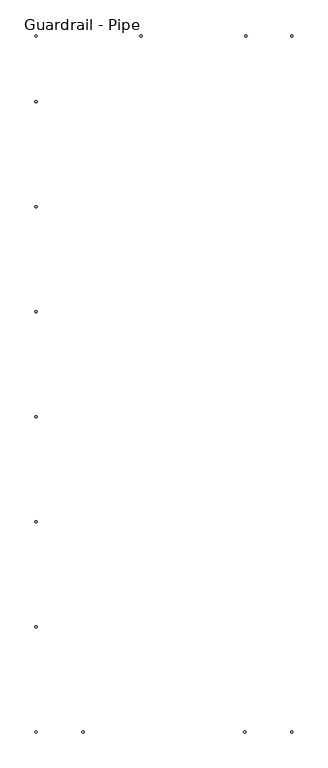
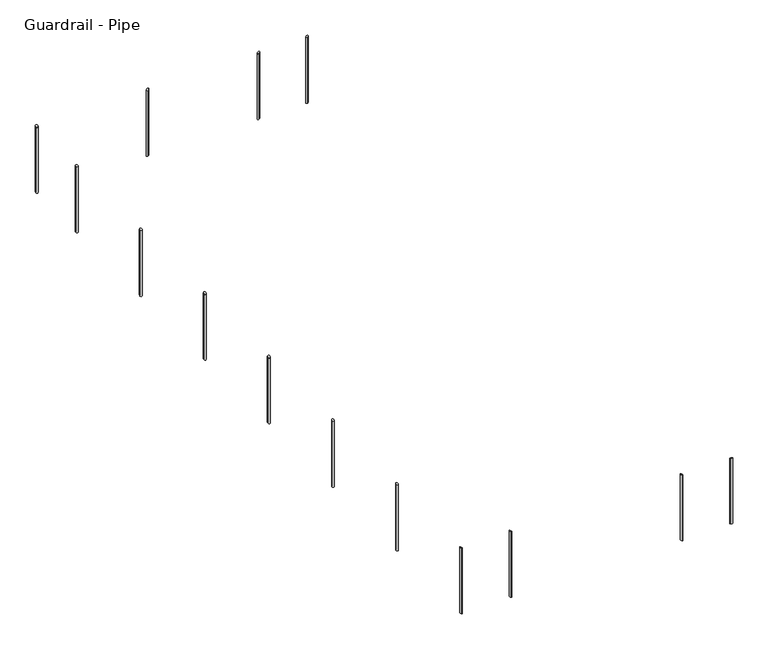
"""IFC4 building model written with IfcOpenShell, lengths in millimetres: railing geometry, Guardrail - Pipe."""

from ifc_helpers import new_model, si_unit, frame, origin, place, context, project, spatial, ellipse_curve, source, transform, mapped, element, save
from ifc_brep_helpers import plane_surface, cylinder_surface, advanced_brep


def guardrail_pipe_e2f870d2(model_context):
    return source(origin(), model_context, "Body", "AdvancedBrep", [
        advanced_brep(
        [(13413.9313551, 29924.3, 8077.2), (13413.9313551, 29924.3, 7315.2), (13413.9313551, 29949.7, 7315.2), (13413.9313551, 29949.7, 8077.2)],
        [
            (0, 1),
            (1, 2, ellipse_curve(frame((13413.9313551, 29937.0, 7315.2), z_axis=(-0.536857935986758, 0.0, 0.8436726596068158), x_axis=(0.8436726596068159, 0.0, 0.536857935986758)), 15.0532317, 12.7)),
            (2, 3),
            (3, 0, ellipse_curve(frame((13413.9313551, 29937.0, 8077.2), z_axis=(0.5368579359867546, 0.0, -0.8436726596068179), x_axis=(0.843672659606818, 0.0, 0.5368579359867547)), 15.0532317, 12.7)),
            (0, 3, ellipse_curve(frame((13413.9313551, 29937.0, 8077.2), z_axis=(0.5368579359867546, 0.0, -0.8436726596068179), x_axis=(0.843672659606818, 0.0, 0.5368579359867547)), 15.0532317, 12.7)),
            (2, 1, ellipse_curve(frame((13413.9313551, 29937.0, 7315.2), z_axis=(-0.536857935986758, 0.0, 0.8436726596068158), x_axis=(0.8436726596068159, 0.0, 0.536857935986758)), 15.0532317, 12.7)),
        ],
        [
            cylinder_surface(frame((13413.9313551, 29937.0, 7086.6), z_axis=(0.0, 0.0, 1.0), x_axis=(0.0, 1.0, 0.0)), 12.7),
            plane_surface(frame((13439.3313551, 29962.4, 8093.3628938), z_axis=(-0.5368579359867546, 0.0, 0.8436726596068179), x_axis=(0.0, -1.0, 0.0))),
            plane_surface(frame((13388.5313551, 29962.4, 7299.0371062), z_axis=(0.536857935986758, 0.0, -0.8436726596068158), x_axis=(0.0, -1.0, 0.0))),
        ],
        [
            (0, [[1, 2, 3, 4]]),
            (0, [[-1, 5, -3, 6]]),
            (1, [[-4, -5]]),
            (2, [[-2, -6]]),
        ],
    ),
        advanced_brep(
        [(12194.7313551, 29924.3, 8077.2), (12194.7313551, 29924.3, 7315.2), (12194.7313551, 29949.7, 7315.2), (12194.7313551, 29949.7, 8077.2)],
        [
            (0, 1),
            (1, 2, ellipse_curve(frame((12194.7313551, 29937.0, 7315.2), z_axis=(-0.536857935986758, 0.0, 0.8436726596068158), x_axis=(0.8436726596068159, 0.0, 0.536857935986758)), 15.0532317, 12.7)),
            (2, 3),
            (3, 0, ellipse_curve(frame((12194.7313551, 29937.0, 8077.2), z_axis=(0.5368579359867546, 0.0, -0.8436726596068179), x_axis=(0.843672659606818, 0.0, 0.5368579359867547)), 15.0532317, 12.7)),
            (0, 3, ellipse_curve(frame((12194.7313551, 29937.0, 8077.2), z_axis=(0.5368579359867546, 0.0, -0.8436726596068179), x_axis=(0.843672659606818, 0.0, 0.5368579359867547)), 15.0532317, 12.7)),
            (2, 1, ellipse_curve(frame((12194.7313551, 29937.0, 7315.2), z_axis=(-0.536857935986758, 0.0, 0.8436726596068158), x_axis=(0.8436726596068159, 0.0, 0.536857935986758)), 15.0532317, 12.7)),
        ],
        [
            cylinder_surface(frame((12194.7313551, 29937.0, 7086.6), z_axis=(0.0, 0.0, 1.0), x_axis=(0.0, 1.0, 0.0)), 12.7),
            plane_surface(frame((12220.1313551, 29962.4, 8093.3628938), z_axis=(-0.5368579359867546, 0.0, 0.8436726596068179), x_axis=(0.0, -1.0, 0.0))),
            plane_surface(frame((12169.3313551, 29962.4, 7299.0371062), z_axis=(0.536857935986758, 0.0, -0.8436726596068158), x_axis=(0.0, -1.0, 0.0))),
        ],
        [
            (0, [[1, 2, 3, 4]]),
            (0, [[-1, 5, -3, 6]]),
            (1, [[-4, -5]]),
            (2, [[-2, -6]]),
        ],
    ),
        advanced_brep(
        [(10988.2313551, 29175.0, 8077.2), (10988.2313551, 29175.0, 7315.2), (10962.8313551, 29175.0, 7315.2), (10962.8313551, 29175.0, 8077.2)],
        [
            (0, 1),
            (1, 2, ellipse_curve(frame((10975.5313551, 29175.0, 7315.2), z_axis=(0.0, -0.536857935986758, 0.8436726596068158), x_axis=(0.0, 0.8436726596068159, 0.536857935986758)), 15.0532317, 12.7)),
            (2, 3),
            (3, 0, ellipse_curve(frame((10975.5313551, 29175.0, 8077.2), z_axis=(0.0, 0.5368579359867546, -0.8436726596068179), x_axis=(0.0, 0.843672659606818, 0.5368579359867547)), 15.0532317, 12.7)),
            (0, 3, ellipse_curve(frame((10975.5313551, 29175.0, 8077.2), z_axis=(0.0, 0.5368579359867546, -0.8436726596068179), x_axis=(0.0, 0.843672659606818, 0.5368579359867547)), 15.0532317, 12.7)),
            (2, 1, ellipse_curve(frame((10975.5313551, 29175.0, 7315.2), z_axis=(0.0, -0.536857935986758, 0.8436726596068158), x_axis=(0.0, 0.8436726596068159, 0.536857935986758)), 15.0532317, 12.7)),
        ],
        [
            cylinder_surface(frame((10975.5313551, 29175.0, 7086.6), z_axis=(0.0, 0.0, 1.0), x_axis=(-1.0, 0.0, 0.0)), 12.7),
            plane_surface(frame((10950.1313551, 29200.4, 8093.3628938), z_axis=(0.0, -0.5368579359867546, 0.8436726596068179), x_axis=(1.0, 0.0, 0.0))),
            plane_surface(frame((10950.1313551, 29149.6, 7299.0371062), z_axis=(0.0, 0.536857935986758, -0.8436726596068158), x_axis=(1.0, 0.0, 0.0))),
        ],
        [
            (0, [[1, 2, 3, 4]]),
            (0, [[-1, 5, -3, 6]]),
            (1, [[-4, -5]]),
            (2, [[-2, -6]]),
        ],
    ),
        advanced_brep(
        [(10988.2313551, 27955.8, 8077.2), (10988.2313551, 27955.8, 7315.2), (10962.8313551, 27955.8, 7315.2), (10962.8313551, 27955.8, 8077.2)],
        [
            (0, 1),
            (1, 2, ellipse_curve(frame((10975.5313551, 27955.8, 7315.2), z_axis=(0.0, -0.536857935986758, 0.8436726596068158), x_axis=(0.0, 0.8436726596068159, 0.536857935986758)), 15.0532317, 12.7)),
            (2, 3),
            (3, 0, ellipse_curve(frame((10975.5313551, 27955.8, 8077.2), z_axis=(0.0, 0.5368579359867546, -0.8436726596068179), x_axis=(0.0, 0.843672659606818, 0.5368579359867547)), 15.0532317, 12.7)),
            (0, 3, ellipse_curve(frame((10975.5313551, 27955.8, 8077.2), z_axis=(0.0, 0.5368579359867546, -0.8436726596068179), x_axis=(0.0, 0.843672659606818, 0.5368579359867547)), 15.0532317, 12.7)),
            (2, 1, ellipse_curve(frame((10975.5313551, 27955.8, 7315.2), z_axis=(0.0, -0.536857935986758, 0.8436726596068158), x_axis=(0.0, 0.8436726596068159, 0.536857935986758)), 15.0532317, 12.7)),
        ],
        [
            cylinder_surface(frame((10975.5313551, 27955.8, 7086.6), z_axis=(0.0, 0.0, 1.0), x_axis=(-1.0, 0.0, 0.0)), 12.7),
            plane_surface(frame((10950.1313551, 27981.2, 8093.3628938), z_axis=(0.0, -0.5368579359867546, 0.8436726596068179), x_axis=(1.0, 0.0, 0.0))),
            plane_surface(frame((10950.1313551, 27930.4, 7299.0371062), z_axis=(0.0, 0.536857935986758, -0.8436726596068158), x_axis=(1.0, 0.0, 0.0))),
        ],
        [
            (0, [[1, 2, 3, 4]]),
            (0, [[-1, 5, -3, 6]]),
            (1, [[-4, -5]]),
            (2, [[-2, -6]]),
        ],
    ),
        advanced_brep(
        [(10988.2313551, 26736.6, 8077.2), (10988.2313551, 26736.6, 7315.2), (10962.8313551, 26736.6, 7315.2), (10962.8313551, 26736.6, 8077.2)],
        [
            (0, 1),
            (1, 2, ellipse_curve(frame((10975.5313551, 26736.6, 7315.2), z_axis=(0.0, -0.536857935986758, 0.8436726596068158), x_axis=(0.0, 0.8436726596068159, 0.536857935986758)), 15.0532317, 12.7)),
            (2, 3),
            (3, 0, ellipse_curve(frame((10975.5313551, 26736.6, 8077.2), z_axis=(0.0, 0.5368579359867546, -0.8436726596068179), x_axis=(0.0, 0.843672659606818, 0.5368579359867547)), 15.0532317, 12.7)),
            (0, 3, ellipse_curve(frame((10975.5313551, 26736.6, 8077.2), z_axis=(0.0, 0.5368579359867546, -0.8436726596068179), x_axis=(0.0, 0.843672659606818, 0.5368579359867547)), 15.0532317, 12.7)),
            (2, 1, ellipse_curve(frame((10975.5313551, 26736.6, 7315.2), z_axis=(0.0, -0.536857935986758, 0.8436726596068158), x_axis=(0.0, 0.8436726596068159, 0.536857935986758)), 15.0532317, 12.7)),
        ],
        [
            cylinder_surface(frame((10975.5313551, 26736.6, 7086.6), z_axis=(0.0, 0.0, 1.0), x_axis=(-1.0, 0.0, 0.0)), 12.7),
            plane_surface(frame((10950.1313551, 26762.0, 8093.3628938), z_axis=(0.0, -0.5368579359867546, 0.8436726596068179), x_axis=(1.0, 0.0, 0.0))),
            plane_surface(frame((10950.1313551, 26711.2, 7299.0371062), z_axis=(0.0, 0.536857935986758, -0.8436726596068158), x_axis=(1.0, 0.0, 0.0))),
        ],
        [
            (0, [[1, 2, 3, 4]]),
            (0, [[-1, 5, -3, 6]]),
            (1, [[-4, -5]]),
            (2, [[-2, -6]]),
        ],
    ),
        advanced_brep(
        [(10988.2313551, 25517.4, 8077.2), (10988.2313551, 25517.4, 7315.2), (10962.8313551, 25517.4, 7315.2), (10962.8313551, 25517.4, 8077.2)],
        [
            (0, 1),
            (1, 2, ellipse_curve(frame((10975.5313551, 25517.4, 7315.2), z_axis=(0.0, -0.536857935986758, 0.8436726596068158), x_axis=(0.0, 0.8436726596068159, 0.536857935986758)), 15.0532317, 12.7)),
            (2, 3),
            (3, 0, ellipse_curve(frame((10975.5313551, 25517.4, 8077.2), z_axis=(0.0, 0.5368579359867546, -0.8436726596068179), x_axis=(0.0, 0.843672659606818, 0.5368579359867547)), 15.0532317, 12.7)),
            (0, 3, ellipse_curve(frame((10975.5313551, 25517.4, 8077.2), z_axis=(0.0, 0.5368579359867546, -0.8436726596068179), x_axis=(0.0, 0.843672659606818, 0.5368579359867547)), 15.0532317, 12.7)),
            (2, 1, ellipse_curve(frame((10975.5313551, 25517.4, 7315.2), z_axis=(0.0, -0.536857935986758, 0.8436726596068158), x_axis=(0.0, 0.8436726596068159, 0.536857935986758)), 15.0532317, 12.7)),
        ],
        [
            cylinder_surface(frame((10975.5313551, 25517.4, 7086.6), z_axis=(0.0, 0.0, 1.0), x_axis=(-1.0, 0.0, 0.0)), 12.7),
            plane_surface(frame((10950.1313551, 25542.8, 8093.3628938), z_axis=(0.0, -0.5368579359867546, 0.8436726596068179), x_axis=(1.0, 0.0, 0.0))),
            plane_surface(frame((10950.1313551, 25492.0, 7299.0371062), z_axis=(0.0, 0.536857935986758, -0.8436726596068158), x_axis=(1.0, 0.0, 0.0))),
        ],
        [
            (0, [[1, 2, 3, 4]]),
            (0, [[-1, 5, -3, 6]]),
            (1, [[-4, -5]]),
            (2, [[-2, -6]]),
        ],
    ),
        advanced_brep(
        [(10988.2313551, 24298.2, 8077.2), (10988.2313551, 24298.2, 7315.2), (10962.8313551, 24298.2, 7315.2), (10962.8313551, 24298.2, 8077.2)],
        [
            (0, 1),
            (1, 2, ellipse_curve(frame((10975.5313551, 24298.2, 7315.2), z_axis=(0.0, -0.536857935986758, 0.8436726596068158), x_axis=(0.0, 0.8436726596068159, 0.536857935986758)), 15.0532317, 12.7)),
            (2, 3),
            (3, 0, ellipse_curve(frame((10975.5313551, 24298.2, 8077.2), z_axis=(0.0, 0.5368579359867546, -0.8436726596068179), x_axis=(0.0, 0.843672659606818, 0.5368579359867547)), 15.0532317, 12.7)),
            (0, 3, ellipse_curve(frame((10975.5313551, 24298.2, 8077.2), z_axis=(0.0, 0.5368579359867546, -0.8436726596068179), x_axis=(0.0, 0.843672659606818, 0.5368579359867547)), 15.0532317, 12.7)),
            (2, 1, ellipse_curve(frame((10975.5313551, 24298.2, 7315.2), z_axis=(0.0, -0.536857935986758, 0.8436726596068158), x_axis=(0.0, 0.8436726596068159, 0.536857935986758)), 15.0532317, 12.7)),
        ],
        [
            cylinder_surface(frame((10975.5313551, 24298.2, 7086.6), z_axis=(0.0, 0.0, 1.0), x_axis=(-1.0, 0.0, 0.0)), 12.7),
            plane_surface(frame((10950.1313551, 24323.6, 8093.3628938), z_axis=(0.0, -0.5368579359867546, 0.8436726596068179), x_axis=(1.0, 0.0, 0.0))),
            plane_surface(frame((10950.1313551, 24272.8, 7299.0371062), z_axis=(0.0, 0.536857935986758, -0.8436726596068158), x_axis=(1.0, 0.0, 0.0))),
        ],
        [
            (0, [[1, 2, 3, 4]]),
            (0, [[-1, 5, -3, 6]]),
            (1, [[-4, -5]]),
            (2, [[-2, -6]]),
        ],
    ),
        advanced_brep(
        [(10988.2313551, 23079.0, 8077.2), (10988.2313551, 23079.0, 7315.2), (10962.8313551, 23079.0, 7315.2), (10962.8313551, 23079.0, 8077.2)],
        [
            (0, 1),
            (1, 2, ellipse_curve(frame((10975.5313551, 23079.0, 7315.2), z_axis=(0.0, -0.536857935986758, 0.8436726596068158), x_axis=(0.0, 0.8436726596068159, 0.536857935986758)), 15.0532317, 12.7)),
            (2, 3),
            (3, 0, ellipse_curve(frame((10975.5313551, 23079.0, 8077.2), z_axis=(0.0, 0.5368579359867546, -0.8436726596068179), x_axis=(0.0, 0.843672659606818, 0.5368579359867547)), 15.0532317, 12.7)),
            (0, 3, ellipse_curve(frame((10975.5313551, 23079.0, 8077.2), z_axis=(0.0, 0.5368579359867546, -0.8436726596068179), x_axis=(0.0, 0.843672659606818, 0.5368579359867547)), 15.0532317, 12.7)),
            (2, 1, ellipse_curve(frame((10975.5313551, 23079.0, 7315.2), z_axis=(0.0, -0.536857935986758, 0.8436726596068158), x_axis=(0.0, 0.8436726596068159, 0.536857935986758)), 15.0532317, 12.7)),
        ],
        [
            cylinder_surface(frame((10975.5313551, 23079.0, 7086.6), z_axis=(0.0, 0.0, 1.0), x_axis=(-1.0, 0.0, 0.0)), 12.7),
            plane_surface(frame((10950.1313551, 23104.4, 8093.3628938), z_axis=(0.0, -0.5368579359867546, 0.8436726596068179), x_axis=(1.0, 0.0, 0.0))),
            plane_surface(frame((10950.1313551, 23053.6, 7299.0371062), z_axis=(0.0, 0.536857935986758, -0.8436726596068158), x_axis=(1.0, 0.0, 0.0))),
        ],
        [
            (0, [[1, 2, 3, 4]]),
            (0, [[-1, 5, -3, 6]]),
            (1, [[-4, -5]]),
            (2, [[-2, -6]]),
        ],
    ),
        advanced_brep(
        [(13935.4313551, 21859.8, 8077.2), (13935.4313551, 21859.8, 7315.2), (13960.8313551, 21859.8, 7315.2), (13960.8313551, 21859.8, 8077.2)],
        [
            (0, 1),
            (1, 2, ellipse_curve(frame((13948.1313551, 21859.8, 7315.2), z_axis=(0.0, 0.536857935986758, 0.8436726596068158), x_axis=(0.0, -0.8436726596068159, 0.536857935986758)), 15.0532317, 12.7)),
            (2, 3),
            (3, 0, ellipse_curve(frame((13948.1313551, 21859.8, 8077.2), z_axis=(0.0, -0.5368579359867546, -0.8436726596068179), x_axis=(0.0, -0.843672659606818, 0.5368579359867547)), 15.0532317, 12.7)),
            (0, 3, ellipse_curve(frame((13948.1313551, 21859.8, 8077.2), z_axis=(0.0, -0.5368579359867546, -0.8436726596068179), x_axis=(0.0, -0.843672659606818, 0.5368579359867547)), 15.0532317, 12.7)),
            (2, 1, ellipse_curve(frame((13948.1313551, 21859.8, 7315.2), z_axis=(0.0, 0.536857935986758, 0.8436726596068158), x_axis=(0.0, -0.8436726596068159, 0.536857935986758)), 15.0532317, 12.7)),
        ],
        [
            cylinder_surface(frame((13948.1313551, 21859.8, 7086.6), z_axis=(0.0, 0.0, 1.0), x_axis=(1.0, 0.0, 0.0)), 12.7),
            plane_surface(frame((13973.5313551, 21834.4, 8093.3628938), z_axis=(0.0, 0.5368579359867546, 0.8436726596068179), x_axis=(-1.0, 0.0, 0.0))),
            plane_surface(frame((13973.5313551, 21885.2, 7299.0371062), z_axis=(0.0, -0.536857935986758, -0.8436726596068158), x_axis=(-1.0, 0.0, 0.0))),
        ],
        [
            (0, [[1, 2, 3, 4]]),
            (0, [[-1, 5, -3, 6]]),
            (1, [[-4, -5]]),
            (2, [[-2, -6]]),
        ],
    ),
        advanced_brep(
        [(13948.1313551, 29924.3, 8077.2), (13948.1313551, 29924.3, 7315.2), (13948.1313551, 29949.7, 7315.2), (13948.1313551, 29949.7, 8077.2)],
        [
            (0, 1),
            (1, 2, ellipse_curve(frame((13948.1313551, 29937.0, 7315.2), z_axis=(-0.536857935986758, 0.0, 0.8436726596068158), x_axis=(0.8436726596068159, 0.0, 0.536857935986758)), 15.0532317, 12.7)),
            (2, 3),
            (3, 0, ellipse_curve(frame((13948.1313551, 29937.0, 8077.2), z_axis=(0.5368579359867546, 0.0, -0.8436726596068179), x_axis=(0.843672659606818, 0.0, 0.5368579359867547)), 15.0532317, 12.7)),
            (0, 3, ellipse_curve(frame((13948.1313551, 29937.0, 8077.2), z_axis=(0.5368579359867546, 0.0, -0.8436726596068179), x_axis=(0.843672659606818, 0.0, 0.5368579359867547)), 15.0532317, 12.7)),
            (2, 1, ellipse_curve(frame((13948.1313551, 29937.0, 7315.2), z_axis=(-0.536857935986758, 0.0, 0.8436726596068158), x_axis=(0.8436726596068159, 0.0, 0.536857935986758)), 15.0532317, 12.7)),
        ],
        [
            cylinder_surface(frame((13948.1313551, 29937.0, 7086.6), z_axis=(0.0, 0.0, 1.0), x_axis=(0.0, 1.0, 0.0)), 12.7),
            plane_surface(frame((13973.5313551, 29962.4, 8093.3628938), z_axis=(-0.5368579359867546, 0.0, 0.8436726596068179), x_axis=(0.0, -1.0, 0.0))),
            plane_surface(frame((13922.7313551, 29962.4, 7299.0371062), z_axis=(0.536857935986758, 0.0, -0.8436726596068158), x_axis=(0.0, -1.0, 0.0))),
        ],
        [
            (0, [[1, 2, 3, 4]]),
            (0, [[-1, 5, -3, 6]]),
            (1, [[-4, -5]]),
            (2, [[-2, -6]]),
        ],
    ),
        advanced_brep(
        [(10988.2313551, 29937.0, 8077.2), (10988.2313551, 29937.0, 7315.2), (10962.8313551, 29937.0, 7315.2), (10962.8313551, 29937.0, 8077.2)],
        [
            (0, 1),
            (1, 2, ellipse_curve(frame((10975.5313551, 29937.0, 7315.2), z_axis=(0.0, -0.536857935986758, 0.8436726596068158), x_axis=(0.0, 0.8436726596068159, 0.536857935986758)), 15.0532317, 12.7)),
            (2, 3),
            (3, 0, ellipse_curve(frame((10975.5313551, 29937.0, 8077.2), z_axis=(0.0, 0.5368579359867546, -0.8436726596068179), x_axis=(0.0, 0.843672659606818, 0.5368579359867547)), 15.0532317, 12.7)),
            (0, 3, ellipse_curve(frame((10975.5313551, 29937.0, 8077.2), z_axis=(0.0, 0.5368579359867546, -0.8436726596068179), x_axis=(0.0, 0.843672659606818, 0.5368579359867547)), 15.0532317, 12.7)),
            (2, 1, ellipse_curve(frame((10975.5313551, 29937.0, 7315.2), z_axis=(0.0, -0.536857935986758, 0.8436726596068158), x_axis=(0.0, 0.8436726596068159, 0.536857935986758)), 15.0532317, 12.7)),
        ],
        [
            cylinder_surface(frame((10975.5313551, 29937.0, 7086.6), z_axis=(0.0, 0.0, 1.0), x_axis=(-1.0, 0.0, 0.0)), 12.7),
            plane_surface(frame((10950.1313551, 29962.4, 8093.3628938), z_axis=(0.0, -0.5368579359867546, 0.8436726596068179), x_axis=(1.0, 0.0, 0.0))),
            plane_surface(frame((10950.1313551, 29911.6, 7299.0371062), z_axis=(0.0, 0.536857935986758, -0.8436726596068158), x_axis=(1.0, 0.0, 0.0))),
        ],
        [
            (0, [[1, 2, 3, 4]]),
            (0, [[-1, 5, -3, 6]]),
            (1, [[-4, -5]]),
            (2, [[-2, -6]]),
        ],
    ),
        advanced_brep(
        [(10975.5313551, 21872.5, 8077.2), (10975.5313551, 21872.5, 7315.2), (10975.5313551, 21847.1, 7315.2), (10975.5313551, 21847.1, 8077.2)],
        [
            (0, 1),
            (1, 2, ellipse_curve(frame((10975.5313551, 21859.8, 7315.2), z_axis=(0.536857935986758, 0.0, 0.8436726596068158), x_axis=(-0.8436726596068159, 0.0, 0.536857935986758)), 15.0532317, 12.7)),
            (2, 3),
            (3, 0, ellipse_curve(frame((10975.5313551, 21859.8, 8077.2), z_axis=(-0.5368579359867546, 0.0, -0.8436726596068179), x_axis=(-0.843672659606818, 0.0, 0.5368579359867547)), 15.0532317, 12.7)),
            (0, 3, ellipse_curve(frame((10975.5313551, 21859.8, 8077.2), z_axis=(-0.5368579359867546, 0.0, -0.8436726596068179), x_axis=(-0.843672659606818, 0.0, 0.5368579359867547)), 15.0532317, 12.7)),
            (2, 1, ellipse_curve(frame((10975.5313551, 21859.8, 7315.2), z_axis=(0.536857935986758, 0.0, 0.8436726596068158), x_axis=(-0.8436726596068159, 0.0, 0.536857935986758)), 15.0532317, 12.7)),
        ],
        [
            cylinder_surface(frame((10975.5313551, 21859.8, 7086.6), z_axis=(0.0, 0.0, 1.0), x_axis=(0.0, -1.0, 0.0)), 12.7),
            plane_surface(frame((10950.1313551, 21834.4, 8093.3628938), z_axis=(0.5368579359867546, 0.0, 0.8436726596068179), x_axis=(0.0, 1.0, 0.0))),
            plane_surface(frame((11000.9313551, 21834.4, 7299.0371062), z_axis=(-0.536857935986758, 0.0, -0.8436726596068158), x_axis=(0.0, 1.0, 0.0))),
        ],
        [
            (0, [[1, 2, 3, 4]]),
            (0, [[-1, 5, -3, 6]]),
            (1, [[-4, -5]]),
            (2, [[-2, -6]]),
        ],
    ),
        advanced_brep(
        [(13402.0313551, 21872.5, 8077.2), (13402.0313551, 21872.5, 7315.2), (13402.0313551, 21847.1, 7315.2), (13402.0313551, 21847.1, 8077.2)],
        [
            (0, 1),
            (1, 2, ellipse_curve(frame((13402.0313551, 21859.8, 7315.2), z_axis=(0.536857935986758, 0.0, 0.8436726596068158), x_axis=(-0.8436726596068159, 0.0, 0.536857935986758)), 15.0532317, 12.7)),
            (2, 3),
            (3, 0, ellipse_curve(frame((13402.0313551, 21859.8, 8077.2), z_axis=(-0.5368579359867546, 0.0, -0.8436726596068179), x_axis=(-0.843672659606818, 0.0, 0.5368579359867547)), 15.0532317, 12.7)),
            (0, 3, ellipse_curve(frame((13402.0313551, 21859.8, 8077.2), z_axis=(-0.5368579359867546, 0.0, -0.8436726596068179), x_axis=(-0.843672659606818, 0.0, 0.5368579359867547)), 15.0532317, 12.7)),
            (2, 1, ellipse_curve(frame((13402.0313551, 21859.8, 7315.2), z_axis=(0.536857935986758, 0.0, 0.8436726596068158), x_axis=(-0.8436726596068159, 0.0, 0.536857935986758)), 15.0532317, 12.7)),
        ],
        [
            cylinder_surface(frame((13402.0313551, 21859.8, 7086.6), z_axis=(0.0, 0.0, 1.0), x_axis=(0.0, -1.0, 0.0)), 12.7),
            plane_surface(frame((13376.6313551, 21834.4, 8093.3628938), z_axis=(0.5368579359867546, 0.0, 0.8436726596068179), x_axis=(0.0, 1.0, 0.0))),
            plane_surface(frame((13427.4313551, 21834.4, 7299.0371062), z_axis=(-0.536857935986758, 0.0, -0.8436726596068158), x_axis=(0.0, 1.0, 0.0))),
        ],
        [
            (0, [[1, 2, 3, 4]]),
            (0, [[-1, 5, -3, 6]]),
            (1, [[-4, -5]]),
            (2, [[-2, -6]]),
        ],
    ),
        advanced_brep(
        [(11521.6313551, 21872.5, 8077.2), (11521.6313551, 21872.5, 7315.2), (11521.6313551, 21847.1, 7315.2), (11521.6313551, 21847.1, 8077.2)],
        [
            (0, 1),
            (1, 2, ellipse_curve(frame((11521.6313551, 21859.8, 7315.2), z_axis=(0.536857935986758, 0.0, 0.8436726596068158), x_axis=(-0.8436726596068159, 0.0, 0.536857935986758)), 15.0532317, 12.7)),
            (2, 3),
            (3, 0, ellipse_curve(frame((11521.6313551, 21859.8, 8077.2), z_axis=(-0.5368579359867546, 0.0, -0.8436726596068179), x_axis=(-0.843672659606818, 0.0, 0.5368579359867547)), 15.0532317, 12.7)),
            (0, 3, ellipse_curve(frame((11521.6313551, 21859.8, 8077.2), z_axis=(-0.5368579359867546, 0.0, -0.8436726596068179), x_axis=(-0.843672659606818, 0.0, 0.5368579359867547)), 15.0532317, 12.7)),
            (2, 1, ellipse_curve(frame((11521.6313551, 21859.8, 7315.2), z_axis=(0.536857935986758, 0.0, 0.8436726596068158), x_axis=(-0.8436726596068159, 0.0, 0.536857935986758)), 15.0532317, 12.7)),
        ],
        [
            cylinder_surface(frame((11521.6313551, 21859.8, 7086.6), z_axis=(0.0, 0.0, 1.0), x_axis=(0.0, -1.0, 0.0)), 12.7),
            plane_surface(frame((11496.2313551, 21834.4, 8093.3628938), z_axis=(0.5368579359867546, 0.0, 0.8436726596068179), x_axis=(0.0, 1.0, 0.0))),
            plane_surface(frame((11547.0313551, 21834.4, 7299.0371062), z_axis=(-0.536857935986758, 0.0, -0.8436726596068158), x_axis=(0.0, 1.0, 0.0))),
        ],
        [
            (0, [[1, 2, 3, 4]]),
            (0, [[-1, 5, -3, 6]]),
            (1, [[-4, -5]]),
            (2, [[-2, -6]]),
        ],
    ),
    ])


if __name__ == "__main__":
    model = new_model("IFC4")
    model_context = context("Model", 3, world=origin())
    ifc_project = project(units=[si_unit("LENGTHUNIT", "METRE", prefix="MILLI")], contexts=[model_context])
    site = spatial("IfcSite", under=ifc_project)
    building = spatial("IfcBuilding", under=site)
    placement = place(None, origin())
    guardrail_pipe_shape = guardrail_pipe_e2f870d2(model_context)
    element("IfcRailing", 1, ObjectType="Guardrail - Pipe", at=placement, inside=building, context=model_context, shape_type="MappedRepresentation", body=[
        mapped(guardrail_pipe_shape, transform((0.0, 0.0, 0.0), x_axis=(1.0, 0.0, 0.0), y_axis=(0.0, 1.0, 0.0), z_axis=(0.0, 0.0, 1.0))),
    ])
    save(model, "model.ifc")
